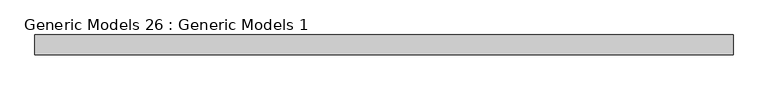
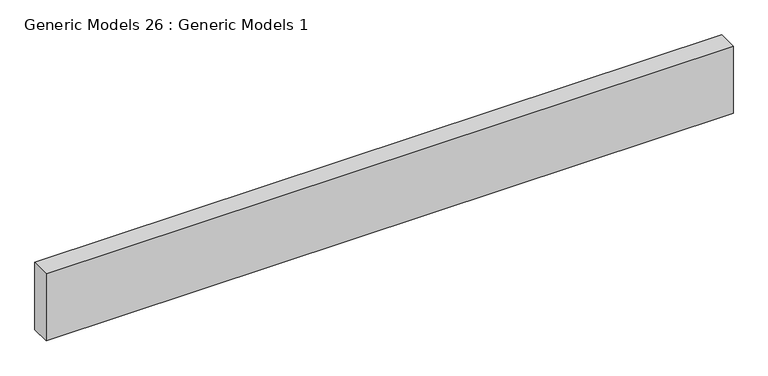
"""IFC4 building model written with IfcOpenShell, lengths in millimetres: proxy geometry, Generic Models 26 : Generic Models 1."""

from ifc_helpers import new_model, si_unit, frame, origin, place, context, project, spatial, polyline, outline, extrude, source, transform, mapped, element, save


def generic_models_26_generic_models_1_0198f28e(model_context):
    return source(origin(), model_context, "Body", "SweptSolid", [
        extrude(outline(polyline([(7162.6263704, 4561.4650592), (7162.6263704, 4599.5650592), (8508.8263704, 4599.5650592), (8508.8263704, 4561.4650592), (7162.6263704, 4561.4650592)])), frame((0.0, 0.0, 126345.696), z_axis=(0.0, 0.0, 1.0), x_axis=(1.0, 0.0, 0.0)), (0.0, 0.0, 1.0), 139.7),
    ])


if __name__ == "__main__":
    model = new_model("IFC4")
    model_context = context("Model", 3, world=origin())
    ifc_project = project(units=[si_unit("LENGTHUNIT", "METRE", prefix="MILLI")], contexts=[model_context])
    site = spatial("IfcSite", under=ifc_project)
    building = spatial("IfcBuilding", under=site)
    placement = place(None, origin())
    generic_models_26_generic_models_1_shape = generic_models_26_generic_models_1_0198f28e(model_context)
    element("IfcBuildingElementProxy", 1, Name="Generic Models 26 : Generic Models 1", ObjectType="Generic Models 26 : Generic Models 1", at=placement, inside=building, context=model_context, shape_type="MappedRepresentation", body=[
        mapped(generic_models_26_generic_models_1_shape, transform((0.0, 0.0, 0.0), x_axis=(1.0, 0.0, 0.0), y_axis=(0.0, 1.0, 0.0), z_axis=(0.0, 0.0, 1.0))),
    ])
    save(model, "model.ifc")

# Revit data of these elements
# Element 1 (IfcBuildingElementProxy, "Generic Models 26 : Generic Models 1")
#   Materials on its faces: "_STRUCTURAL MEMBER (SEE STRUCT. DWGS)"
# Materials
#   "_STRUCTURAL MEMBER (SEE STRUCT. DWGS)": class "Generic", colour RGB 209 182 141, transparency 0, Cost = 0
